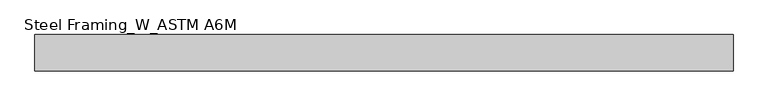
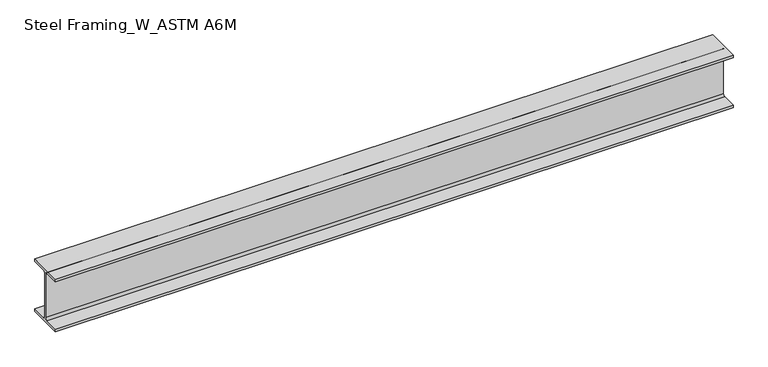
"""IFC4 building model written with IfcOpenShell, lengths in millimetres: beam geometry, Steel Framing_W_ASTM A6M : H_SB_AR_S02_W200x31.3_B6."""

from ifc_helpers import new_model, si_unit, point, frame, frame_2d, origin, place, context, project, spatial, polyline, circle_curve, trimmed, segment, composite_curve, outline, extrude, source, transform, mapped, element, save


def steel_framing_w_astm_a6m_6ea1ca7e(model_context):
    return source(origin(), model_context, "Body", "SweptSolid", [
        extrude(outline(composite_curve([segment(polyline([(67.0, -94.8), (67.0, -105.0), (-67.0, -105.0), (-67.0, -94.8), (-10.775, -94.8)]), True, "CONTINUOUS"), segment(trimmed(circle_curve(frame_2d((-10.775, -87.2)), 7.6), [point((-10.775, -94.8))], [point((-3.175, -87.2))], True, "CARTESIAN"), True, "CONTINUOUS"), segment(polyline([(-3.175, -87.2), (-3.175, 87.2)]), True, "CONTINUOUS"), segment(trimmed(circle_curve(frame_2d((-10.775, 87.2)), 7.6), [point((-3.175, 87.2))], [point((-10.775, 94.8))], True, "CARTESIAN"), True, "CONTINUOUS"), segment(polyline([(-10.775, 94.8), (-67.0, 94.8), (-67.0, 105.0), (67.0, 105.0), (67.0, 94.8), (10.775, 94.8)]), True, "CONTINUOUS"), segment(trimmed(circle_curve(frame_2d((10.775, 87.2)), 7.6), [point((10.775, 94.8))], [point((3.175, 87.2))], True, "CARTESIAN"), True, "CONTINUOUS"), segment(polyline([(3.175, 87.2), (3.175, -87.2)]), True, "CONTINUOUS"), segment(trimmed(circle_curve(frame_2d((10.775, -87.2)), 7.6), [point((3.175, -87.2))], [point((10.775, -94.8))], True, "CARTESIAN"), True, "CONTINUOUS"), segment(polyline([(10.775, -94.8), (67.0, -94.8)]), True, "CONTINUOUS")], self_intersect=False)), frame((-1320.3, 0.0, 0.0), z_axis=(1.0, 0.0, 0.0), x_axis=(0.0, 1.0, 0.0)), (0.0, 0.0, 1.0), 2566.6),
    ])


if __name__ == "__main__":
    model = new_model("IFC4")
    model_context = context("Model", 3, world=origin())
    ifc_project = project(units=[si_unit("LENGTHUNIT", "METRE", prefix="MILLI")], contexts=[model_context])
    site = spatial("IfcSite", under=ifc_project)
    building = spatial("IfcBuilding", under=site)
    placement = place(None, origin())
    steel_framing_w_astm_a6m_shape = steel_framing_w_astm_a6m_6ea1ca7e(model_context)
    element("IfcBeam", 1, ObjectType="Steel Framing_W_ASTM A6M : H_SB_AR_S02_W200x31.3_B6", at=placement, inside=building, context=model_context, shape_type="MappedRepresentation", body=[
        mapped(steel_framing_w_astm_a6m_shape, transform((0.0, 0.0, 0.0), x_axis=(1.0, 0.0, 0.0), y_axis=(0.0, 1.0, 0.0), z_axis=(0.0, 0.0, 1.0))),
    ])
    save(model, "model.ifc")

# Revit data of these elements
# Type "Steel Framing_W_ASTM A6M : H_SB_AR_S02_W200x31.3_B6"
#   Type Mark = "B6"
#   Section Name Key = "W8x21"
#   Width = 13.4 cm
#   Web Thickness = 0.635 cm
#   Web Fillet = 0.76 cm
#   Warping Constant = 40800.0 cm⁶
#   Torsional Moment of Inertia = 11.70 cm⁴
#   Section Area = 39.7 cm²
#   Plastic Modulus weak axis = 93.2 cm³
#   Plastic Modulus strong axis = 334.0 cm³
#   Perimeter = 0.93 m²/m
#   Nominal Weight = 31.30 kgf/m
#   Moment of Inertia weak axis = 407.00 cm⁴
#   Moment of Inertia strong axis = 3130.00 cm⁴
#   Height = 21.0 cm
#   Flange Thickness = 1.02 cm
#   Elastic Modulus weak axis = 60.8 cm³
#   Elastic Modulus strong axis = 298.0 cm³
#   Centroid Vertical = 10.5 cm
#   Centroid Horizontal = 6.7 cm
#   Length [instance default] = 1500 mm
#   Structural Material [instance default] = Steel, 45-345
#   Bolt Spacing = 0
#   Assembly Code = ""
# Element 1 (IfcBeam, "Steel Framing_W_ASTM A6M : H_SB_AR_S02_W200x31.3_B6")
#   Materials on its faces: "Steel, 45-345"
# Materials
#   "Steel, 45-345": class "Metal", colour RGB 189 187 185, transparency 0, Description = "Steel 345 MPa", Cost = 0
